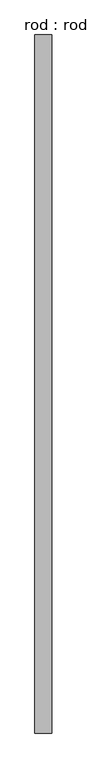
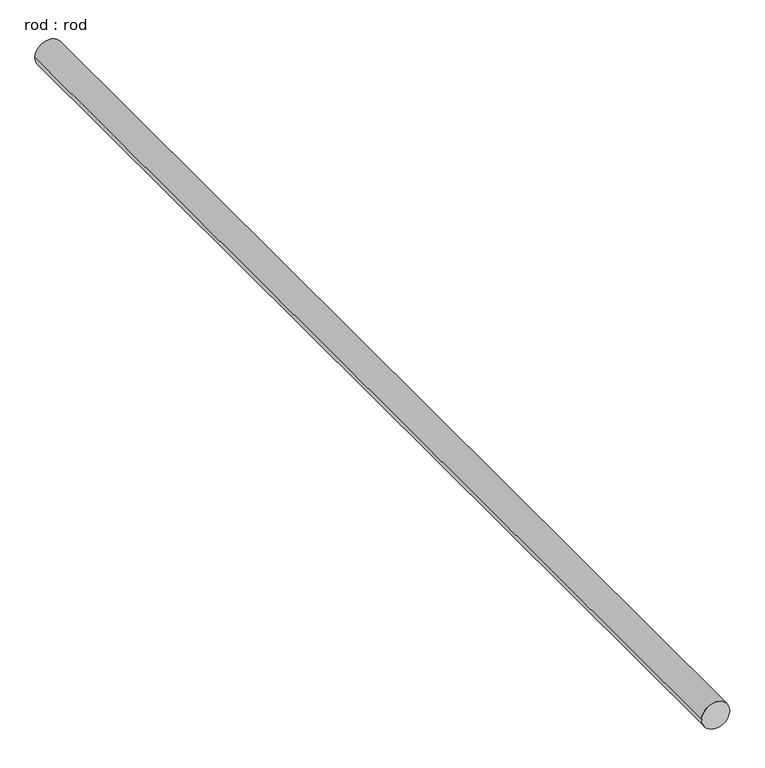
"""IFC4 building model written with IfcOpenShell, lengths in millimetres: proxy geometry, rod : rod."""

from ifc_helpers import new_model, si_unit, point, frame, frame_2d, origin, place, context, project, spatial, circle_curve, trimmed, segment, composite_curve, outline, extrude, source, transform, mapped, element, save


def rod_rod_b5dab0b0(model_context):
    return source(origin(), model_context, "Body", "SweptSolid", [
        extrude(outline(composite_curve([segment(trimmed(circle_curve(frame_2d((0.0108462, 0.0)), 200.0), [point((0.0108462, 200.0))], [point((0.0108462, -200.0))], False, "CARTESIAN"), True, "CONTINUOUS"), segment(trimmed(circle_curve(frame_2d((0.0108462, 0.0)), 200.0), [point((0.0108462, -200.0))], [point((0.0108462, 200.0))], False, "CARTESIAN"), True, "CONTINUOUS")], self_intersect=False)), frame((0.0, -4149.8808048, 0.0), z_axis=(0.0, 1.0, 0.0), x_axis=(0.0, 0.0, 1.0)), (0.0, 0.0, 1.0), 16485.2188402),
    ])


if __name__ == "__main__":
    model = new_model("IFC4")
    model_context = context("Model", 3, world=origin())
    ifc_project = project(units=[si_unit("LENGTHUNIT", "METRE", prefix="MILLI")], contexts=[model_context])
    site = spatial("IfcSite", under=ifc_project)
    building = spatial("IfcBuilding", under=site)
    placement = place(None, origin())
    rod_rod_shape = rod_rod_b5dab0b0(model_context)
    element("IfcBuildingElementProxy", 1, Name="rod : rod", ObjectType="rod : rod", at=placement, inside=building, context=model_context, shape_type="MappedRepresentation", body=[
        mapped(rod_rod_shape, transform((0.0, 0.0, 0.0), x_axis=(1.0, 0.0, 0.0), y_axis=(0.0, 1.0, 0.0), z_axis=(0.0, 0.0, 1.0))),
    ])
    save(model, "model.ifc")

# Revit data of these elements
# Type "rod : rod"
#   Default Elevation = 0
